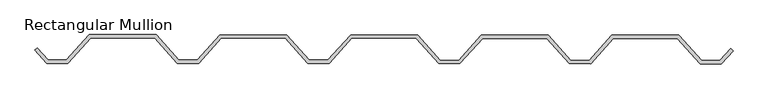
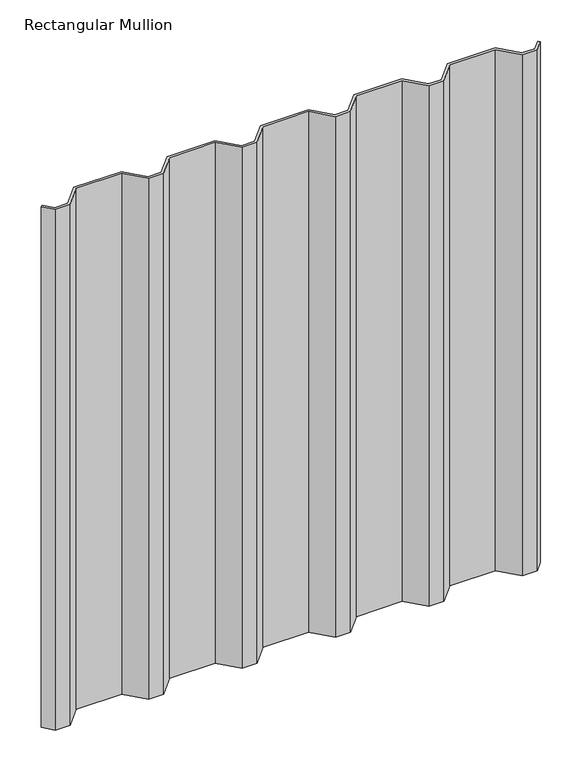
"""IFC4 building model written with IfcOpenShell, lengths in millimetres: member geometry, Rectangular Mullion : Telha Metálica - Trapezoidal."""

import ifcopenshell
import ifcopenshell.guid

model = None  # the IFC model being written
_history = None  # IfcOwnerHistory: only IFC2X3 demands one
_inside = {}  # id of a spatial element -> (the spatial element, [elements in it])
_under = {}  # id of a project, library or spatial element -> (it, [spatial elements below it])
_declared = {}  # id of a project -> (the project, [libraries it declares])
_typed = {}  # id of a type object -> (the type object, [elements of that type])
_made_of = {}  # id of a material, layer set ... -> (it, [elements and type objects made of it])


def new_model(schema):
    """Start an empty IFC model of exactly this schema.

    Asked for "IFC4X3", IfcOpenShell would pick the latest addendum, in which some entities
    have other attributes; the version numbers below select the first issue.
    IFC2X3 requires an IfcOwnerHistory on every rooted entity: one is made here for all.
    """
    global model, _history
    if schema == "IFC4X3":
        model = ifcopenshell.file(schema_version=(4, 3, 0, 0))
    else:
        model = ifcopenshell.file(schema=schema)
    _inside.clear()
    _under.clear()
    _declared.clear()
    _typed.clear()
    _made_of.clear()
    _history = None
    if model.schema == "IFC2X3":
        org = make("IfcOrganization", Name="unknown")
        user = make(
            "IfcPersonAndOrganization",
            ThePerson=make("IfcPerson", FamilyName="unknown"),
            TheOrganization=org,
        )
        app = make(
            "IfcApplication",
            ApplicationDeveloper=org,
            Version="unknown",
            ApplicationFullName="unknown",
            ApplicationIdentifier="unknown",
        )
        _history = make(
            "IfcOwnerHistory",
            OwningUser=user,
            OwningApplication=app,
            ChangeAction="ADDED",
            CreationDate=0,
        )
    return model


def make(cls, **values):
    """One entity of the class cls with the attributes given. An attribute that is None is left unset."""
    return model.create_entity(
        cls, **{name: value for name, value in values.items() if value is not None}
    )


def rooted(cls, **values):
    """An entity with a GlobalId (a new one), such as an element, a storey or a relation."""
    return make(cls, GlobalId=ifcopenshell.guid.new(), OwnerHistory=_history, **values)


def si_unit(unit_type, name, prefix=None):
    """IfcSIUnit, for example si_unit("LENGTHUNIT", "METRE", prefix="MILLI")."""
    return make("IfcSIUnit", UnitType=unit_type, Prefix=prefix, Name=name)


def assignment(units):
    """IfcUnitAssignment: the units of a project."""
    return None if units is None else make("IfcUnitAssignment", Units=units)


def point(xyz):
    """IfcCartesianPoint."""
    return None if xyz is None else make("IfcCartesianPoint", Coordinates=xyz)


def direction(xyz):
    """IfcDirection."""
    return None if xyz is None else make("IfcDirection", DirectionRatios=xyz)


def frame(location, z_axis=None, x_axis=None):
    """IfcAxis2Placement3D, a coordinate frame: its origin and axes. An axis left out is left unset."""
    return make(
        "IfcAxis2Placement3D",
        Location=point(location),
        Axis=direction(z_axis),
        RefDirection=direction(x_axis),
    )


def origin():
    """The frame at (0, 0, 0) with its axes left unset."""
    return frame((0.0, 0.0, 0.0))


def place(relative_to, where):
    """IfcLocalPlacement: puts the frame where relative to a parent placement (None: the world)."""
    return make(
        "IfcLocalPlacement", PlacementRelTo=relative_to, RelativePlacement=where
    )


def context(
    kind, dimensions, precision=None, world=None, true_north=None, identifier=None
):
    """IfcGeometricRepresentationContext, for example the 3D "Model" context."""
    return make(
        "IfcGeometricRepresentationContext",
        ContextIdentifier=identifier,
        ContextType=kind,
        CoordinateSpaceDimension=dimensions,
        Precision=precision,
        WorldCoordinateSystem=world,
        TrueNorth=true_north,
    )


def project(units=None, contexts=None):
    """IfcProject with its units and contexts."""
    return rooted(
        "IfcProject",
        Name="project",
        RepresentationContexts=contexts,
        UnitsInContext=assignment(units),
    )


def spatial(cls, under=None, at=None, **own):
    """A site, building, storey or space (cls), placed at a placement, below another one or the project."""
    s = rooted(cls, ObjectPlacement=at, **own)
    if under is not None:
        _under.setdefault(under.id(), (under, []))[1].append(s)
    return s


def polyline(points):
    """IfcPolyline through the points."""
    return make("IfcPolyline", Points=[point(p) for p in points])


def outline(outer, holes=None, kind="AREA"):
    """IfcArbitraryClosedProfileDef: a profile drawn as a closed curve; with holes, ...WithVoids."""
    if holes is None:
        return make("IfcArbitraryClosedProfileDef", ProfileType=kind, OuterCurve=outer)
    return make(
        "IfcArbitraryProfileDefWithVoids",
        ProfileType=kind,
        OuterCurve=outer,
        InnerCurves=holes,
    )


def extrude(swept, where, along, depth):
    """IfcExtrudedAreaSolid: the profile swept, set in the frame where, extruded along a direction by depth."""
    return make(
        "IfcExtrudedAreaSolid",
        SweptArea=swept,
        Position=where,
        ExtrudedDirection=direction(along),
        Depth=depth,
    )


def shape(context_of_items, identifier, shape_type, items):
    """IfcShapeRepresentation: the items that make up one representation, for example the "Body"."""
    return make(
        "IfcShapeRepresentation",
        ContextOfItems=context_of_items,
        RepresentationIdentifier=identifier,
        RepresentationType=shape_type,
        Items=items,
    )


def source(mapping_origin, context_of_items, identifier, shape_type, items):
    """IfcRepresentationMap: a shape defined once, which mapped items show again and again."""
    return make(
        "IfcRepresentationMap",
        MappingOrigin=mapping_origin,
        MappedRepresentation=shape(context_of_items, identifier, shape_type, items),
    )


def transform(
    local_origin,
    x_axis=None,
    y_axis=None,
    z_axis=None,
    scale=None,
    scale2=None,
    scale3=None,
    uniform=True,
):
    """IfcCartesianTransformationOperator3D, or its non-uniform kind. x_axis, y_axis, z_axis: its Axis1, 2, 3."""
    if uniform:
        return make(
            "IfcCartesianTransformationOperator3D",
            Axis1=direction(x_axis),
            Axis2=direction(y_axis),
            LocalOrigin=point(local_origin),
            Scale=scale,
            Axis3=direction(z_axis),
        )
    return make(
        "IfcCartesianTransformationOperator3DnonUniform",
        Axis1=direction(x_axis),
        Axis2=direction(y_axis),
        LocalOrigin=point(local_origin),
        Scale=scale,
        Axis3=direction(z_axis),
        Scale2=scale2,
        Scale3=scale3,
    )


def mapped(mapping_source, mapping_target):
    """IfcMappedItem: shows the shape of a source again, moved by a transform."""
    return make(
        "IfcMappedItem", MappingSource=mapping_source, MappingTarget=mapping_target
    )


def made_of(thing, what):
    """Note that an element or type object is made of a material, layer set ...; save() writes the relation."""
    if what is not None:
        _made_of.setdefault(what.id(), (what, []))[1].append(thing)
    return thing


def element(
    cls,
    number,
    at=None,
    inside=None,
    cuts=None,
    type_object=None,
    material=None,
    context=None,
    identifier="Body",
    shape_type=None,
    held_by="IfcProductDefinitionShape",
    body=None,
    shapes=None,
    **own,
):
    """One element of the class cls, such as IfcWall. Its Tag is "e" and its number.

    at: its placement. inside: the storey or other place that contains it. cuts: it is an
    opening in that element (IfcRelVoidsElement). A single representation is given by context,
    identifier, shape_type and body (its items); several are given by shapes. held_by: the class
    of the entity that holds the representations. save() writes the other relations.
    """
    e = rooted(cls, Tag="e%d" % number, ObjectPlacement=at, **own)
    if body is not None:
        shapes = [shape(context, identifier, shape_type, body)]
    if shapes is not None:
        e.Representation = make(held_by, Representations=shapes)
    if inside is not None:
        _inside.setdefault(inside.id(), (inside, []))[1].append(e)
    if cuts is not None:
        rooted(
            "IfcRelVoidsElement", RelatingBuildingElement=cuts, RelatedOpeningElement=e
        )
    if type_object is not None:
        _typed.setdefault(type_object.id(), (type_object, []))[1].append(e)
    return made_of(e, material)


def aggregate(whole, parts):
    """IfcRelAggregates: a whole, such as a stair, and the parts it consists of."""
    return rooted("IfcRelAggregates", RelatingObject=whole, RelatedObjects=parts)


def save(model, path):
    """Write the relations noted so far, then the file.

    IfcRelAggregates (storeys below a building ...), IfcRelContainedInSpatialStructure (elements
    in a storey), IfcRelDefinesByType, IfcRelAssociatesMaterial and IfcRelDeclares: one each for
    every whole, place, type object, material and project.
    """
    for whole, parts in _under.values():
        aggregate(whole, parts)
    for where, things in _inside.values():
        rooted(
            "IfcRelContainedInSpatialStructure",
            RelatedElements=things,
            RelatingStructure=where,
        )
    for kind, things in _typed.values():
        rooted("IfcRelDefinesByType", RelatedObjects=things, RelatingType=kind)
    for what, things in _made_of.values():
        rooted("IfcRelAssociatesMaterial", RelatedObjects=things, RelatingMaterial=what)
    for by, libraries in _declared.values():
        rooted("IfcRelDeclares", RelatingContext=by, RelatedDefinitions=libraries)
    model.write(path)


def rectangular_mullion_c1e6517d(model_context):
    return source(origin(), model_context, "Body", "SweptSolid", [
        extrude(outline(polyline([(440.066155, 75.6159987), (344.0661915, 75.6997745), (310.0330432, 37.7294595), (278.0330554, 37.7573848), (244.0662296, 75.7870409), (148.0662661, 75.8708167), (114.0331178, 37.9005018), (82.03313, 37.928427), (48.0663042, 75.9580832), (-47.9336592, 76.041859), (-81.9668075, 38.071544), (-113.9667953, 38.0994693), (-147.9336211, 76.1291254), (-243.9335846, 76.2129012), (-277.9667329, 38.2425863), (-309.9667207, 38.2705115), (-343.9335465, 76.3001677), (-439.93351, 76.3839434), (-473.9666583, 38.4136285), (-505.9666461, 38.4415538), (-523.4905169, 58.0614849), (-519.9464424, 61.5993792), (-503.7267316, 43.439601), (-476.1978461, 43.4155775), (-442.1646978, 81.3858924), (-341.693632, 81.2982149), (-307.7268062, 43.2685587), (-280.1979207, 43.2445352), (-246.1647724, 81.2148502), (-145.6937067, 81.1271726), (-111.7268809, 43.0975165), (-84.1979953, 43.073493), (-50.164847, 81.0438079), (50.3062187, 80.9561304), (84.2730445, 42.9264742), (111.80193, 42.9024508), (145.8350783, 80.8727657), (246.3061441, 80.7850881), (280.2729699, 42.755432), (307.8018554, 42.7314085), (341.8350037, 80.7017235), (442.3060694, 80.6140459), (476.2728952, 42.5843898), (503.8017808, 42.5603663), (520.072301, 60.7131616), (523.6101953, 57.1690871), (506.0329686, 37.5584173), (474.0329808, 37.5863426), (440.066155, 75.6159987)])), frame((0.0, 0.0, -1154.7005384), z_axis=(0.0, 0.0, 1.0), x_axis=(1.0, 0.0, 0.0)), (0.0, 0.0, 1.0), 1154.7005384),
    ])


if __name__ == "__main__":
    model = new_model("IFC4")
    model_context = context("Model", 3, world=origin())
    ifc_project = project(units=[si_unit("LENGTHUNIT", "METRE", prefix="MILLI")], contexts=[model_context])
    site = spatial("IfcSite", under=ifc_project)
    building = spatial("IfcBuilding", under=site)
    placement = place(None, origin())
    rectangular_mullion_shape = rectangular_mullion_c1e6517d(model_context)
    element("IfcMember", 1, ObjectType="Rectangular Mullion : Telha Metálica - Trapezoidal", at=placement, inside=building, context=model_context, shape_type="MappedRepresentation", body=[
        mapped(rectangular_mullion_shape, transform((0.0, 0.0, 0.0), x_axis=(1.0, 0.0, 0.0), y_axis=(0.0, 1.0, 0.0), z_axis=(0.0, 0.0, 1.0))),
    ])
    save(model, "model.ifc")

# Revit data of these elements
# Type "Rectangular Mullion : Telha Metálica - Trapezoidal"
#   built-in parameter 1007322 = 0.0164042 (stored number, unit not read)
# Element 1 (IfcMember, "Rectangular Mullion : Telha Metálica - Trapezoidal")
#   Materials on its faces: "Telha - Metálica"
# Materials
#   "Telha - Metálica": class "Cerâmica", colour RGB 242 242 242, transparency 0, Description = "Interior finish", Cost = 0
